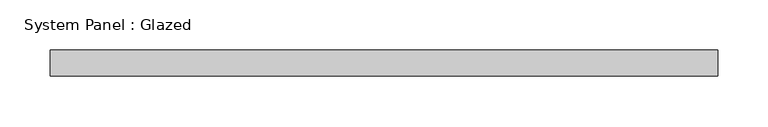
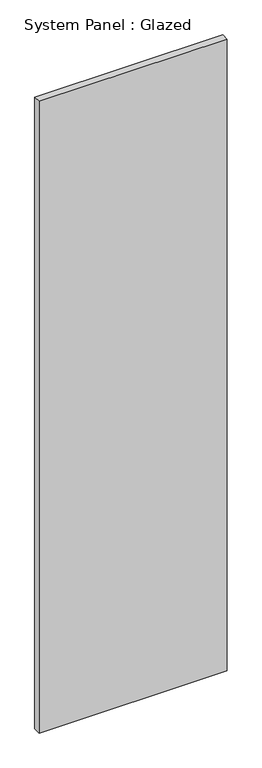
"""IFC4 building model written with IfcOpenShell, lengths in millimetres: plate geometry, System Panel : Glazed."""

import ifcopenshell
import ifcopenshell.guid

model = None  # the IFC model being written
_history = None  # IfcOwnerHistory: only IFC2X3 demands one
_inside = {}  # id of a spatial element -> (the spatial element, [elements in it])
_under = {}  # id of a project, library or spatial element -> (it, [spatial elements below it])
_declared = {}  # id of a project -> (the project, [libraries it declares])
_typed = {}  # id of a type object -> (the type object, [elements of that type])
_made_of = {}  # id of a material, layer set ... -> (it, [elements and type objects made of it])


def new_model(schema):
    """Start an empty IFC model of exactly this schema.

    Asked for "IFC4X3", IfcOpenShell would pick the latest addendum, in which some entities
    have other attributes; the version numbers below select the first issue.
    IFC2X3 requires an IfcOwnerHistory on every rooted entity: one is made here for all.
    """
    global model, _history
    if schema == "IFC4X3":
        model = ifcopenshell.file(schema_version=(4, 3, 0, 0))
    else:
        model = ifcopenshell.file(schema=schema)
    _inside.clear()
    _under.clear()
    _declared.clear()
    _typed.clear()
    _made_of.clear()
    _history = None
    if model.schema == "IFC2X3":
        org = make("IfcOrganization", Name="unknown")
        user = make(
            "IfcPersonAndOrganization",
            ThePerson=make("IfcPerson", FamilyName="unknown"),
            TheOrganization=org,
        )
        app = make(
            "IfcApplication",
            ApplicationDeveloper=org,
            Version="unknown",
            ApplicationFullName="unknown",
            ApplicationIdentifier="unknown",
        )
        _history = make(
            "IfcOwnerHistory",
            OwningUser=user,
            OwningApplication=app,
            ChangeAction="ADDED",
            CreationDate=0,
        )
    return model


def make(cls, **values):
    """One entity of the class cls with the attributes given. An attribute that is None is left unset."""
    return model.create_entity(
        cls, **{name: value for name, value in values.items() if value is not None}
    )


def rooted(cls, **values):
    """An entity with a GlobalId (a new one), such as an element, a storey or a relation."""
    return make(cls, GlobalId=ifcopenshell.guid.new(), OwnerHistory=_history, **values)


def si_unit(unit_type, name, prefix=None):
    """IfcSIUnit, for example si_unit("LENGTHUNIT", "METRE", prefix="MILLI")."""
    return make("IfcSIUnit", UnitType=unit_type, Prefix=prefix, Name=name)


def assignment(units):
    """IfcUnitAssignment: the units of a project."""
    return None if units is None else make("IfcUnitAssignment", Units=units)


def point(xyz):
    """IfcCartesianPoint."""
    return None if xyz is None else make("IfcCartesianPoint", Coordinates=xyz)


def direction(xyz):
    """IfcDirection."""
    return None if xyz is None else make("IfcDirection", DirectionRatios=xyz)


def frame(location, z_axis=None, x_axis=None):
    """IfcAxis2Placement3D, a coordinate frame: its origin and axes. An axis left out is left unset."""
    return make(
        "IfcAxis2Placement3D",
        Location=point(location),
        Axis=direction(z_axis),
        RefDirection=direction(x_axis),
    )


def origin():
    """The frame at (0, 0, 0) with its axes left unset."""
    return frame((0.0, 0.0, 0.0))


def origin_with_axes():
    """The frame at (0, 0, 0) with the z axis (0, 0, 1) and the x axis (1, 0, 0) written out."""
    return frame((0.0, 0.0, 0.0), z_axis=(0.0, 0.0, 1.0), x_axis=(1.0, 0.0, 0.0))


def place(relative_to, where):
    """IfcLocalPlacement: puts the frame where relative to a parent placement (None: the world)."""
    return make(
        "IfcLocalPlacement", PlacementRelTo=relative_to, RelativePlacement=where
    )


def context(
    kind, dimensions, precision=None, world=None, true_north=None, identifier=None
):
    """IfcGeometricRepresentationContext, for example the 3D "Model" context."""
    return make(
        "IfcGeometricRepresentationContext",
        ContextIdentifier=identifier,
        ContextType=kind,
        CoordinateSpaceDimension=dimensions,
        Precision=precision,
        WorldCoordinateSystem=world,
        TrueNorth=true_north,
    )


def project(units=None, contexts=None):
    """IfcProject with its units and contexts."""
    return rooted(
        "IfcProject",
        Name="project",
        RepresentationContexts=contexts,
        UnitsInContext=assignment(units),
    )


def spatial(cls, under=None, at=None, **own):
    """A site, building, storey or space (cls), placed at a placement, below another one or the project."""
    s = rooted(cls, ObjectPlacement=at, **own)
    if under is not None:
        _under.setdefault(under.id(), (under, []))[1].append(s)
    return s


def polyline(points):
    """IfcPolyline through the points."""
    return make("IfcPolyline", Points=[point(p) for p in points])


def outline(outer, holes=None, kind="AREA"):
    """IfcArbitraryClosedProfileDef: a profile drawn as a closed curve; with holes, ...WithVoids."""
    if holes is None:
        return make("IfcArbitraryClosedProfileDef", ProfileType=kind, OuterCurve=outer)
    return make(
        "IfcArbitraryProfileDefWithVoids",
        ProfileType=kind,
        OuterCurve=outer,
        InnerCurves=holes,
    )


def extrude(swept, where, along, depth):
    """IfcExtrudedAreaSolid: the profile swept, set in the frame where, extruded along a direction by depth."""
    return make(
        "IfcExtrudedAreaSolid",
        SweptArea=swept,
        Position=where,
        ExtrudedDirection=direction(along),
        Depth=depth,
    )


def shape(context_of_items, identifier, shape_type, items):
    """IfcShapeRepresentation: the items that make up one representation, for example the "Body"."""
    return make(
        "IfcShapeRepresentation",
        ContextOfItems=context_of_items,
        RepresentationIdentifier=identifier,
        RepresentationType=shape_type,
        Items=items,
    )


def source(mapping_origin, context_of_items, identifier, shape_type, items):
    """IfcRepresentationMap: a shape defined once, which mapped items show again and again."""
    return make(
        "IfcRepresentationMap",
        MappingOrigin=mapping_origin,
        MappedRepresentation=shape(context_of_items, identifier, shape_type, items),
    )


def transform(
    local_origin,
    x_axis=None,
    y_axis=None,
    z_axis=None,
    scale=None,
    scale2=None,
    scale3=None,
    uniform=True,
):
    """IfcCartesianTransformationOperator3D, or its non-uniform kind. x_axis, y_axis, z_axis: its Axis1, 2, 3."""
    if uniform:
        return make(
            "IfcCartesianTransformationOperator3D",
            Axis1=direction(x_axis),
            Axis2=direction(y_axis),
            LocalOrigin=point(local_origin),
            Scale=scale,
            Axis3=direction(z_axis),
        )
    return make(
        "IfcCartesianTransformationOperator3DnonUniform",
        Axis1=direction(x_axis),
        Axis2=direction(y_axis),
        LocalOrigin=point(local_origin),
        Scale=scale,
        Axis3=direction(z_axis),
        Scale2=scale2,
        Scale3=scale3,
    )


def mapped(mapping_source, mapping_target):
    """IfcMappedItem: shows the shape of a source again, moved by a transform."""
    return make(
        "IfcMappedItem", MappingSource=mapping_source, MappingTarget=mapping_target
    )


def made_of(thing, what):
    """Note that an element or type object is made of a material, layer set ...; save() writes the relation."""
    if what is not None:
        _made_of.setdefault(what.id(), (what, []))[1].append(thing)
    return thing


def element(
    cls,
    number,
    at=None,
    inside=None,
    cuts=None,
    type_object=None,
    material=None,
    context=None,
    identifier="Body",
    shape_type=None,
    held_by="IfcProductDefinitionShape",
    body=None,
    shapes=None,
    **own,
):
    """One element of the class cls, such as IfcWall. Its Tag is "e" and its number.

    at: its placement. inside: the storey or other place that contains it. cuts: it is an
    opening in that element (IfcRelVoidsElement). A single representation is given by context,
    identifier, shape_type and body (its items); several are given by shapes. held_by: the class
    of the entity that holds the representations. save() writes the other relations.
    """
    e = rooted(cls, Tag="e%d" % number, ObjectPlacement=at, **own)
    if body is not None:
        shapes = [shape(context, identifier, shape_type, body)]
    if shapes is not None:
        e.Representation = make(held_by, Representations=shapes)
    if inside is not None:
        _inside.setdefault(inside.id(), (inside, []))[1].append(e)
    if cuts is not None:
        rooted(
            "IfcRelVoidsElement", RelatingBuildingElement=cuts, RelatedOpeningElement=e
        )
    if type_object is not None:
        _typed.setdefault(type_object.id(), (type_object, []))[1].append(e)
    return made_of(e, material)


def aggregate(whole, parts):
    """IfcRelAggregates: a whole, such as a stair, and the parts it consists of."""
    return rooted("IfcRelAggregates", RelatingObject=whole, RelatedObjects=parts)


def save(model, path):
    """Write the relations noted so far, then the file.

    IfcRelAggregates (storeys below a building ...), IfcRelContainedInSpatialStructure (elements
    in a storey), IfcRelDefinesByType, IfcRelAssociatesMaterial and IfcRelDeclares: one each for
    every whole, place, type object, material and project.
    """
    for whole, parts in _under.values():
        aggregate(whole, parts)
    for where, things in _inside.values():
        rooted(
            "IfcRelContainedInSpatialStructure",
            RelatedElements=things,
            RelatingStructure=where,
        )
    for kind, things in _typed.values():
        rooted("IfcRelDefinesByType", RelatedObjects=things, RelatingType=kind)
    for what, things in _made_of.values():
        rooted("IfcRelAssociatesMaterial", RelatedObjects=things, RelatingMaterial=what)
    for by, libraries in _declared.values():
        rooted("IfcRelDeclares", RelatingContext=by, RelatedDefinitions=libraries)
    model.write(path)


def system_panel_glazed_baf84a5d(model_context):
    return source(origin(), model_context, "Body", "SweptSolid", [
        extrude(outline(polyline([(330.2, -44.45), (-330.2, -44.45), (-330.2, -19.05), (330.2, -19.05), (330.2, -44.45)])), origin_with_axes(), (0.0, 0.0, 1.0), 2343.15),
    ])


if __name__ == "__main__":
    model = new_model("IFC4")
    model_context = context("Model", 3, world=origin())
    ifc_project = project(units=[si_unit("LENGTHUNIT", "METRE", prefix="MILLI")], contexts=[model_context])
    site = spatial("IfcSite", under=ifc_project)
    building = spatial("IfcBuilding", under=site)
    placement = place(None, origin())
    system_panel_glazed_shape = system_panel_glazed_baf84a5d(model_context)
    element("IfcPlate", 1, ObjectType="System Panel : Glazed", at=placement, inside=building, context=model_context, shape_type="MappedRepresentation", body=[
        mapped(system_panel_glazed_shape, transform((0.0, 0.0, 0.0), x_axis=(1.0, 0.0, 0.0), y_axis=(0.0, 1.0, 0.0), z_axis=(0.0, 0.0, 1.0))),
    ])
    save(model, "model.ifc")

# Revit data of these elements
# Type "System Panel : Glazed"
#   Construction Type Id = "GSP4R"
#   Analytic Construction = "1/8 in Pilkington single glazing"
#   Visual Light Transmittance = 0.9
#   Solar Heat Gain Coefficient = 0.86
#   Heat Transfer Coefficient (U) = 1.18115 BTU/(h·ft²·°F)
#   Define Thermal Properties by = 1
# Element 1 (IfcPlate, "System Panel : Glazed")
#   Materials on its faces: "Glass"
# Materials
#   "Glass": class "Glass", colour RGB 0 128 192, transparency 0.75, Description = "Soda Lime Glass", Cost = 0
